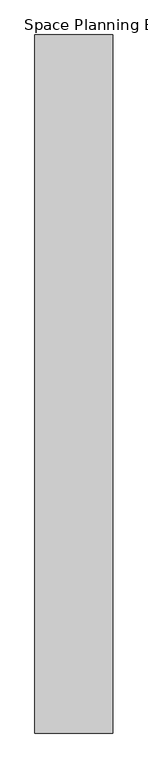
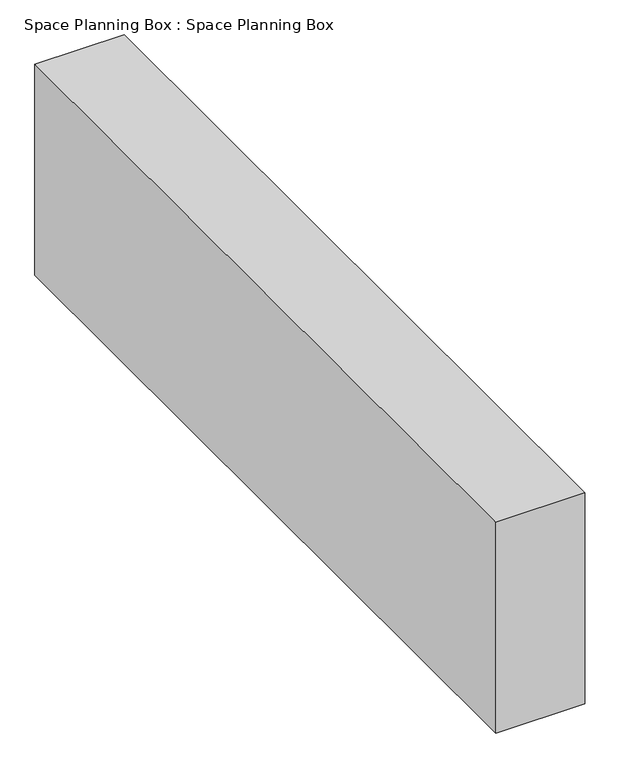
"""IFC4 building model written with IfcOpenShell, lengths in millimetres: proxy geometry, Space Planning Box : Space Planning Box."""

from ifc_helpers import new_model, si_unit, origin, origin_with_axes, place, context, project, spatial, polyline, outline, extrude, source, transform, mapped, element, save


def space_planning_box_space_planning_box_03407eb8(model_context):
    return source(origin(), model_context, "Body", "SweptSolid", [
        extrude(outline(polyline([(1200.0, 10750.0), (1200.0, -10750.0), (-1200.0, -10750.0), (-1200.0, 10750.0), (1200.0, 10750.0)])), origin_with_axes(), (0.0, 0.0, 1.0), 6000.0),
    ])


if __name__ == "__main__":
    model = new_model("IFC4")
    model_context = context("Model", 3, world=origin())
    ifc_project = project(units=[si_unit("LENGTHUNIT", "METRE", prefix="MILLI")], contexts=[model_context])
    site = spatial("IfcSite", under=ifc_project)
    building = spatial("IfcBuilding", under=site)
    placement = place(None, origin())
    space_planning_box_space_planning_box_shape = space_planning_box_space_planning_box_03407eb8(model_context)
    element("IfcBuildingElementProxy", 1, Name="Space Planning Box : Space Planning Box", ObjectType="Space Planning Box : Space Planning Box", at=placement, inside=building, context=model_context, shape_type="MappedRepresentation", body=[
        mapped(space_planning_box_space_planning_box_shape, transform((0.0, 0.0, 0.0), x_axis=(1.0, 0.0, 0.0), y_axis=(0.0, 1.0, 0.0), z_axis=(0.0, 0.0, 1.0))),
    ])
    save(model, "model.ifc")

# Revit data of these elements
# Type "Space Planning Box : Space Planning Box"
#   Type Comments = "..."
#   Room Name [instance default] = "?"
#   Assembly Code = "..."
#   Width [instance default] = 1524 mm
#   Program Area [instance default] = 0 m²
#   Length [instance default] = 1524 mm
#   Height [instance default] = 1524 mm
#   Area [instance default] = 2.32258 m²
#   Fill Color [instance default] = Cyan
#   Default Elevation = 0
# Element 1 (IfcBuildingElementProxy, "Space Planning Box : Space Planning Box")
#   Room Name = "Corridor"
#   Width = 2400 mm
#   Length = 21500 mm
#   Height = 6000 mm
#   Area = 51.6 m²
#   Fill Color = Lavender
#   Materials on its faces: "Lavender"
# Materials
#   "Cyan": class "Generic", colour RGB 0 255 255, transparency 0.2, Cost = 0
#   "Lavender": class "Generic", colour RGB 186 85 211, transparency 0.2, Cost = 0
